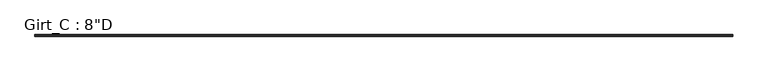
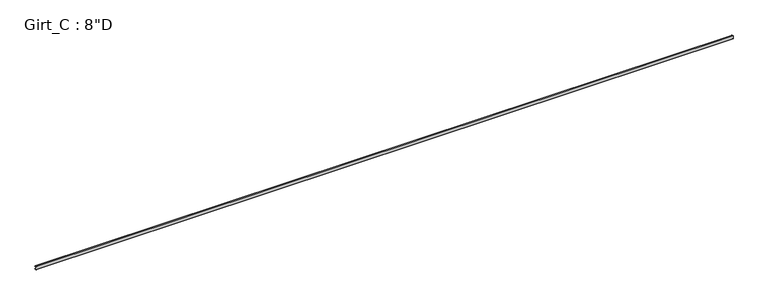
"""IFC4 building model written with IfcOpenShell, lengths in millimetres: beam geometry."""

from ifc_helpers import new_model, si_unit, point, frame, frame_2d, origin, place, context, project, spatial, polyline, circle_curve, trimmed, segment, composite_curve, outline, extrude, source, transform, mapped, element, save


def beam_c287abb1(model_context):
    return source(origin(), model_context, "Body", "SweptSolid", [
        extrude(outline(composite_curve([segment(polyline([(87.5109375, 101.6), (99.7560415, 87.0068534), (97.6278742, 85.221109), (86.2154765, 98.821875), (3.3005807, 98.821875)]), True, "CONTINUOUS"), segment(trimmed(circle_curve(frame_2d((3.3741066, 96.8381931)), 1.9850441), [point((3.3005807, 98.821875))], [point((1.3890625, 96.8381931))], True, "CARTESIAN"), True, "CONTINUOUS"), segment(polyline([(1.3890625, 96.8381931), (1.3890625, -96.8389339)]), True, "CONTINUOUS"), segment(trimmed(circle_curve(frame_2d((3.3748024, -96.8389339)), 1.9857399), [point((1.3890625, -96.8389339))], [point((3.2694106, -98.821875))], True, "CARTESIAN"), True, "CONTINUOUS"), segment(polyline([(3.2694106, -98.821875), (86.2154765, -98.821875), (97.6510975, -85.1934327), (99.7792647, -86.979177), (87.5109375, -101.6), (3.3734375, -101.6)]), True, "CONTINUOUS"), segment(trimmed(circle_curve(frame_2d((3.3734375, -96.8375)), 4.7625), [point((3.3734375, -101.6))], [point((-1.3890625, -96.8375))], False, "CARTESIAN"), True, "CONTINUOUS"), segment(polyline([(-1.3890625, -96.8375), (-1.3890625, 96.8375)]), True, "CONTINUOUS"), segment(trimmed(circle_curve(frame_2d((3.3734375, 96.8375)), 4.7625), [point((-1.3890625, 96.8375))], [point((3.3734375, 101.6))], False, "CARTESIAN"), True, "CONTINUOUS"), segment(polyline([(3.3734375, 101.6), (87.5109375, 101.6)]), True, "CONTINUOUS")], self_intersect=False)), frame((-21958.3, 0.0, 0.0), z_axis=(1.0, 0.0, 0.0), x_axis=(0.0, 1.0, 0.0)), (0.0, 0.0, 1.0), 43891.2),
    ])


if __name__ == "__main__":
    model = new_model("IFC4")
    model_context = context("Model", 3, world=origin())
    ifc_project = project(units=[si_unit("LENGTHUNIT", "METRE", prefix="MILLI")], contexts=[model_context])
    site = spatial("IfcSite", under=ifc_project)
    building = spatial("IfcBuilding", under=site)
    placement = place(None, origin())
    beam_shape = beam_c287abb1(model_context)
    element("IfcBeam", 1, ObjectType="Girt_C : 8\"D", at=placement, inside=building, context=model_context, shape_type="MappedRepresentation", body=[
        mapped(beam_shape, transform((0.0, 0.0, 0.0), x_axis=(1.0, 0.0, 0.0), y_axis=(0.0, 1.0, 0.0), z_axis=(0.0, 0.0, 1.0))),
    ])
    save(model, "model.ifc")

# Revit data of these elements
# Type "Girt_C : 8\"D"
#   half leg = 0' - 1 3/4"
#   Web_Thickness = 0' - 0 7/64"
#   Length [instance default] = 10' - 0"
#   Leg_1 = 0' - 3 1/2"
#   Height = 0' - 8"
#   Structural Material [instance default] = none
# Element 1 (IfcBeam, "Girt_C : 8\"D")
#   Structural Material = CEE' SECTION (8.0x3.5C - SEE STRUCT. DWGS)
#   Materials on its faces: "CEE' SECTION (8.0x3.5C - SEE STRUCT. DWGS)"
# Materials
#   "CEE' SECTION (8.0x3.5C - SEE STRUCT. DWGS)": class "Metal", colour RGB 137 146 153, transparency 0, Description = "Steel, mill finish", Cost = 0
